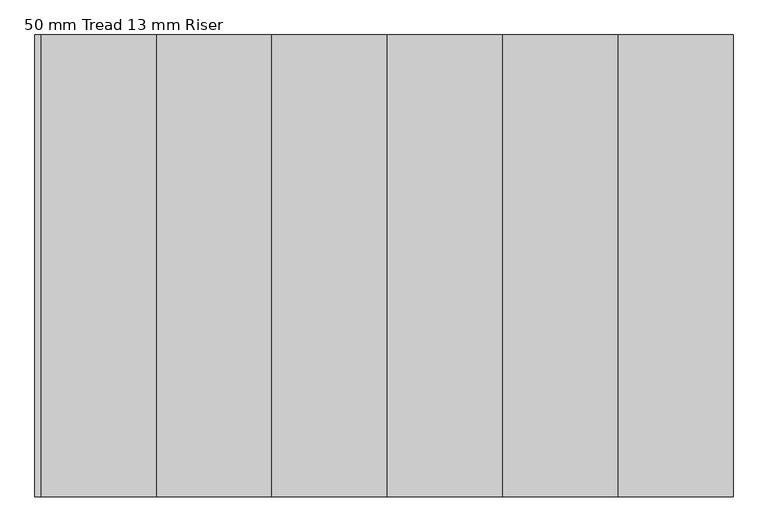
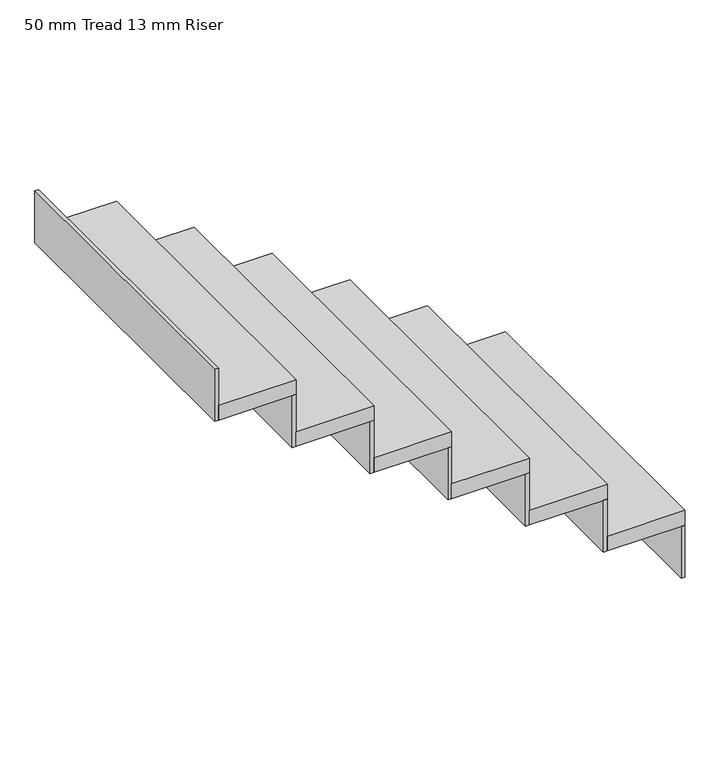
"""IFC4 building model written with IfcOpenShell, lengths in millimetres: stair flight geometry, 50 mm Tread 13 mm Riser."""

from ifc_helpers import new_model, si_unit, frame, origin, place, context, project, spatial, polyline, outline, extrude, source, transform, mapped, element, save


def stair_flight_50_mm_tread_13_mm_riser_627438fb(model_context):
    return source(origin(), model_context, "Body", "SweptSolid", [
        extrude(outline(polyline([(30300.5737371, 990.5195288), (30313.0737371, 990.5195288), (30313.0737371, -9.4804712), (30300.5737371, -9.4804712), (30300.5737371, 990.5195288)])), frame((0.0, 0.0, 1714.7058824), z_axis=(0.0, 0.0, 1.0), x_axis=(1.0, 0.0, 0.0)), (0.0, 0.0, 1.0), 176.4705882),
        extrude(outline(polyline([(30063.0737371, -9.4804712), (30063.0737371, 990.5195288), (30313.0737371, 990.5195288), (30313.0737371, -9.4804712), (30063.0737371, -9.4804712)])), frame((0.0, 0.0, 1891.1764706), z_axis=(0.0, 0.0, 1.0), x_axis=(1.0, 0.0, 0.0)), (0.0, 0.0, 1.0), 50.0),
        extrude(outline(polyline([(30050.5737371, 990.5195288), (30063.0737371, 990.5195288), (30063.0737371, -9.4804712), (30050.5737371, -9.4804712), (30050.5737371, 990.5195288)])), frame((0.0, 0.0, 1891.1764706), z_axis=(0.0, 0.0, 1.0), x_axis=(1.0, 0.0, 0.0)), (0.0, 0.0, 1.0), 176.4705882),
        extrude(outline(polyline([(29813.0737371, -9.4804712), (29813.0737371, 990.5195288), (30063.0737371, 990.5195288), (30063.0737371, -9.4804712), (29813.0737371, -9.4804712)])), frame((0.0, 0.0, 2067.6470588), z_axis=(0.0, 0.0, 1.0), x_axis=(1.0, 0.0, 0.0)), (0.0, 0.0, 1.0), 50.0),
        extrude(outline(polyline([(29800.5737371, 990.5195288), (29813.0737371, 990.5195288), (29813.0737371, -9.4804712), (29800.5737371, -9.4804712), (29800.5737371, 990.5195288)])), frame((0.0, 0.0, 2067.6470588), z_axis=(0.0, 0.0, 1.0), x_axis=(1.0, 0.0, 0.0)), (0.0, 0.0, 1.0), 176.4705882),
        extrude(outline(polyline([(29563.0737371, -9.4804712), (29563.0737371, 990.5195288), (29813.0737371, 990.5195288), (29813.0737371, -9.4804712), (29563.0737371, -9.4804712)])), frame((0.0, 0.0, 2244.1176471), z_axis=(0.0, 0.0, 1.0), x_axis=(1.0, 0.0, 0.0)), (0.0, 0.0, 1.0), 50.0),
        extrude(outline(polyline([(29550.5737371, 990.5195288), (29563.0737371, 990.5195288), (29563.0737371, -9.4804712), (29550.5737371, -9.4804712), (29550.5737371, 990.5195288)])), frame((0.0, 0.0, 2244.1176471), z_axis=(0.0, 0.0, 1.0), x_axis=(1.0, 0.0, 0.0)), (0.0, 0.0, 1.0), 176.4705882),
        extrude(outline(polyline([(29313.0737371, -9.4804712), (29313.0737371, 990.5195288), (29563.0737371, 990.5195288), (29563.0737371, -9.4804712), (29313.0737371, -9.4804712)])), frame((0.0, 0.0, 2420.5882353), z_axis=(0.0, 0.0, 1.0), x_axis=(1.0, 0.0, 0.0)), (0.0, 0.0, 1.0), 50.0),
        extrude(outline(polyline([(29300.5737371, 990.5195288), (29313.0737371, 990.5195288), (29313.0737371, -9.4804712), (29300.5737371, -9.4804712), (29300.5737371, 990.5195288)])), frame((0.0, 0.0, 2420.5882353), z_axis=(0.0, 0.0, 1.0), x_axis=(1.0, 0.0, 0.0)), (0.0, 0.0, 1.0), 176.4705882),
        extrude(outline(polyline([(29063.0737371, -9.4804712), (29063.0737371, 990.5195288), (29313.0737371, 990.5195288), (29313.0737371, -9.4804712), (29063.0737371, -9.4804712)])), frame((0.0, 0.0, 2597.0588235), z_axis=(0.0, 0.0, 1.0), x_axis=(1.0, 0.0, 0.0)), (0.0, 0.0, 1.0), 50.0),
        extrude(outline(polyline([(29050.5737371, 990.5195288), (29063.0737371, 990.5195288), (29063.0737371, -9.4804712), (29050.5737371, -9.4804712), (29050.5737371, 990.5195288)])), frame((0.0, 0.0, 2597.0588235), z_axis=(0.0, 0.0, 1.0), x_axis=(1.0, 0.0, 0.0)), (0.0, 0.0, 1.0), 176.4705882),
        extrude(outline(polyline([(28800.5737371, 990.5195288), (28813.0737371, 990.5195288), (28813.0737371, -9.4804712), (28800.5737371, -9.4804712), (28800.5737371, 990.5195288)])), frame((0.0, 0.0, 2773.5294118), z_axis=(0.0, 0.0, 1.0), x_axis=(1.0, 0.0, 0.0)), (0.0, 0.0, 1.0), 176.4705882),
        extrude(outline(polyline([(28813.0737371, -9.4804712), (28813.0737371, 990.5195288), (29063.0737371, 990.5195288), (29063.0737371, -9.4804712), (28813.0737371, -9.4804712)])), frame((0.0, 0.0, 2773.5294118), z_axis=(0.0, 0.0, 1.0), x_axis=(1.0, 0.0, 0.0)), (0.0, 0.0, 1.0), 50.0),
    ])


if __name__ == "__main__":
    model = new_model("IFC4")
    model_context = context("Model", 3, world=origin())
    ifc_project = project(units=[si_unit("LENGTHUNIT", "METRE", prefix="MILLI")], contexts=[model_context])
    site = spatial("IfcSite", under=ifc_project)
    building = spatial("IfcBuilding", under=site)
    placement = place(None, origin())
    stair_flight_50_mm_tread_13_mm_riser_shape = stair_flight_50_mm_tread_13_mm_riser_627438fb(model_context)
    element("IfcStairFlight", 1, ObjectType="50 mm Tread 13 mm Riser", at=placement, inside=building, context=model_context, shape_type="MappedRepresentation", body=[
        mapped(stair_flight_50_mm_tread_13_mm_riser_shape, transform((0.0, 0.0, 0.0), x_axis=(1.0, 0.0, 0.0), y_axis=(0.0, 1.0, 0.0), z_axis=(0.0, 0.0, 1.0))),
    ])
    save(model, "model.ifc")
